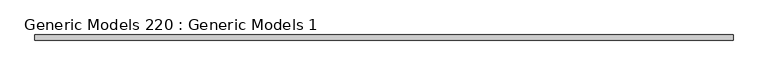
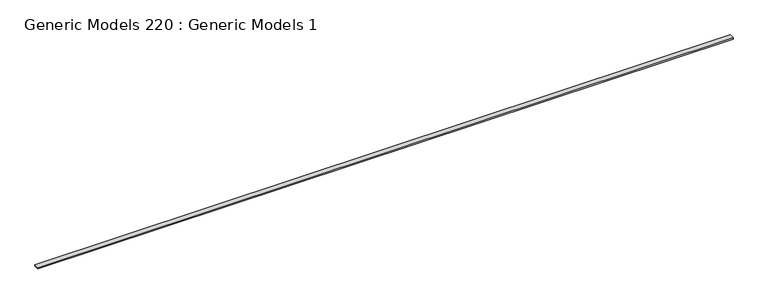
"""IFC4 building model written with IfcOpenShell, lengths in millimetres: proxy geometry, Generic Models 220 : Generic Models 1."""

from ifc_helpers import new_model, si_unit, frame, origin, place, context, project, spatial, polyline, outline, extrude, source, transform, mapped, element, save


def generic_models_220_generic_models_1_46bebbfd(model_context):
    return source(origin(), model_context, "Body", "SweptSolid", [
        extrude(outline(polyline([(-20998.9733045, -29322.5735041), (-20998.9733045, -29182.8735041), (-1948.9733045, -29182.8735041), (-1948.9733045, -29322.5735041), (-20998.9733045, -29322.5735041)])), frame((0.0, 0.0, 127066.3735933), z_axis=(0.0, 0.0, 1.0), x_axis=(1.0, 0.0, 0.0)), (0.0, 0.0, 1.0), 38.1),
    ])


if __name__ == "__main__":
    model = new_model("IFC4")
    model_context = context("Model", 3, world=origin())
    ifc_project = project(units=[si_unit("LENGTHUNIT", "METRE", prefix="MILLI")], contexts=[model_context])
    site = spatial("IfcSite", under=ifc_project)
    building = spatial("IfcBuilding", under=site)
    placement = place(None, origin())
    generic_models_220_generic_models_1_shape = generic_models_220_generic_models_1_46bebbfd(model_context)
    element("IfcBuildingElementProxy", 1, Name="Generic Models 220 : Generic Models 1", ObjectType="Generic Models 220 : Generic Models 1", at=placement, inside=building, context=model_context, shape_type="MappedRepresentation", body=[
        mapped(generic_models_220_generic_models_1_shape, transform((0.0, 0.0, 0.0), x_axis=(1.0, 0.0, 0.0), y_axis=(0.0, 1.0, 0.0), z_axis=(0.0, 0.0, 1.0))),
    ])
    save(model, "model.ifc")

# Revit data of these elements
# Element 1 (IfcBuildingElementProxy, "Generic Models 220 : Generic Models 1")
#   Materials on its faces: "_2X BLOCKING AS REQUIRED"
# Materials
#   "_2X BLOCKING AS REQUIRED": class "Generic", colour RGB 177 130 114, transparency 0, Cost = 0
